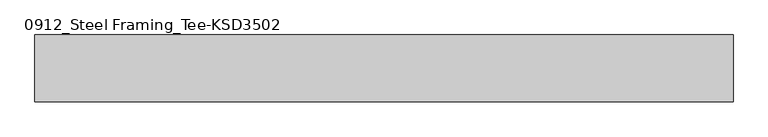
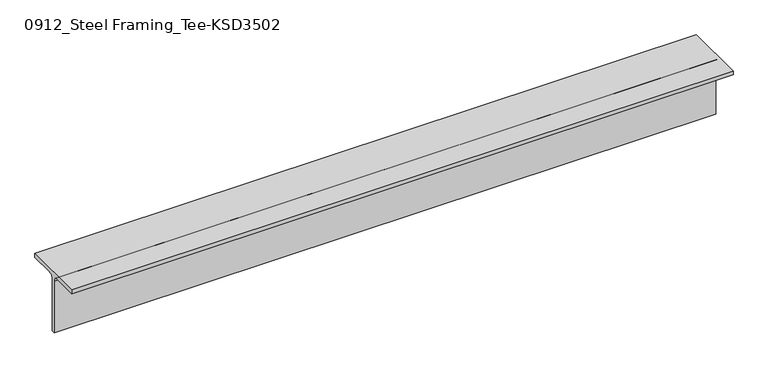
"""IFC4 building model written with IfcOpenShell, lengths in millimetres: member geometry, 0912_Steel Framing_Tee-KSD3502 : H_SB_ASB_CT-150x150x6.5x9."""

from ifc_helpers import new_model, si_unit, point, frame, frame_2d, origin, place, context, project, spatial, polyline, circle_curve, trimmed, segment, composite_curve, outline, extrude, source, transform, mapped, element, save


def member_0912_steel_framing_tee_ksd3502_66338f04(model_context):
    return source(origin(), model_context, "Body", "SweptSolid", [
        extrude(outline(composite_curve([segment(polyline([(75.0, 75.0), (75.0, 66.0), (16.25, 66.0)]), True, "CONTINUOUS"), segment(trimmed(circle_curve(frame_2d((16.25, 53.0)), 13.0), [point((16.25, 66.0))], [point((3.25, 53.0))], True, "CARTESIAN"), True, "CONTINUOUS"), segment(polyline([(3.25, 53.0), (3.25, -75.0), (-3.25, -75.0), (-3.25, 53.0)]), True, "CONTINUOUS"), segment(trimmed(circle_curve(frame_2d((-16.25, 53.0)), 13.0), [point((-3.25, 53.0))], [point((-16.25, 66.0))], True, "CARTESIAN"), True, "CONTINUOUS"), segment(polyline([(-16.25, 66.0), (-75.0, 66.0), (-75.0, 75.0), (75.0, 75.0)]), True, "CONTINUOUS")], self_intersect=False)), frame((-860.2, 0.0, 0.0), z_axis=(1.0, 0.0, 0.0), x_axis=(0.0, 1.0, 0.0)), (0.0, 0.0, 1.0), 1561.9),
    ])


if __name__ == "__main__":
    model = new_model("IFC4")
    model_context = context("Model", 3, world=origin())
    ifc_project = project(units=[si_unit("LENGTHUNIT", "METRE", prefix="MILLI")], contexts=[model_context])
    site = spatial("IfcSite", under=ifc_project)
    building = spatial("IfcBuilding", under=site)
    placement = place(None, origin())
    member_0912_steel_framing_tee_ksd3502_shape = member_0912_steel_framing_tee_ksd3502_66338f04(model_context)
    element("IfcMember", 1, ObjectType="0912_Steel Framing_Tee-KSD3502 : H_SB_ASB_CT-150x150x6.5x9", at=placement, inside=building, context=model_context, shape_type="MappedRepresentation", body=[
        mapped(member_0912_steel_framing_tee_ksd3502_shape, transform((0.0, 0.0, 0.0), x_axis=(1.0, 0.0, 0.0), y_axis=(0.0, 1.0, 0.0), z_axis=(0.0, 0.0, 1.0))),
    ])
    save(model, "model.ifc")

# Revit data of these elements
# Type "0912_Steel Framing_Tee-KSD3502 : H_SB_ASB_CT-150x150x6.5x9"
#   H_WM Code_1 = "S01AA003-00001 | Main Steel Structure Fabrication Work | Shelter/Building | Light Steel - Standard (30KG/M>Weight) | Material: (   )"
#   H_WM Code_2 = "S03AA029-00001 | Main Steel Structure Erection Work | Shelter/Building | Light Steel (30KG/M>Weight) | Material: (   )"
#   H_WM Code_3 = "S01AA010-00001 | Main Steel Structure Fabrication Work | Shelter/Building | Steel Painting/Coating | for Non-Fireproofed Steel Surface, Surface Preparation, Primer, Second & Final Coat | Material: (   )"
#   H_Q'ty Cal Type Tag = "SB-Q2"
#   Width = 15.0 cm
#   Web Thickness = 0.65 cm
#   Web Fillet = 1.3 cm
#   Section Area = 23.39 cm²
#   Perimeter = 0.60 m²/m
#   Nominal Weight = 18.40 kgf/m
#   Height = 15.0 cm
#   Flange Thickness = 0.9 cm
#   Centroid Vertical = 7.5 cm
#   Centroid Horizontal = 7.5 cm
#   Length [instance default] = 1.5000 m
#   Structural Material [instance default] = Steel, 45-345
#   Warping Constant = (empty or 0)
#   Torsional Moment of Inertia = 0
#   Section Name Key = ""
#   Plastic Modulus weak axis = 0
#   Plastic Modulus strong axis = 0
#   Moment of Inertia weak axis = 0
#   Moment of Inertia strong axis = 0
#   Elastic Modulus weak axis = 0
#   Elastic Modulus strong axis = 0
#   Bolt Spacing = 0
#   Assembly Code = ""
# Element 1 (IfcMember, "0912_Steel Framing_Tee-KSD3502 : H_SB_ASB_CT-150x150x6.5x9")
#   Structural Material = none
# Materials
#   "Steel, 45-345": class "Metal", colour RGB 189 187 185, transparency 0, Description = "Steel 345 MPa", Cost = 0
